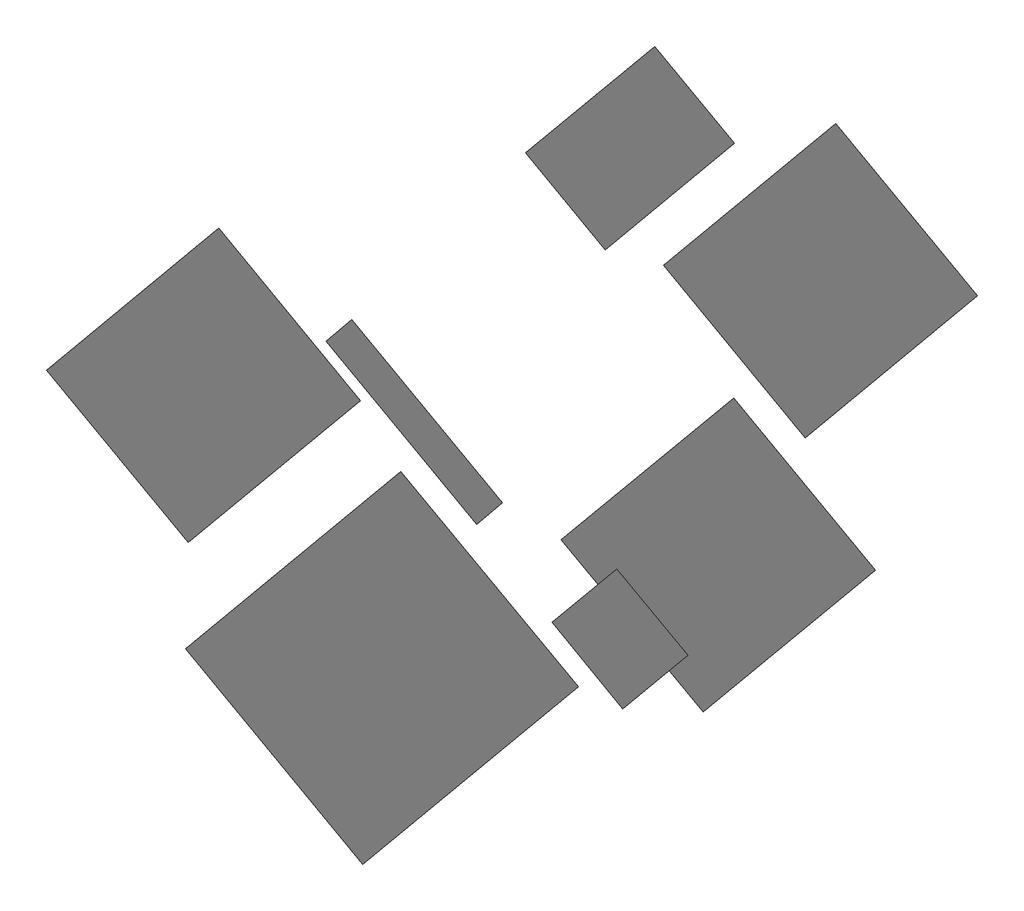
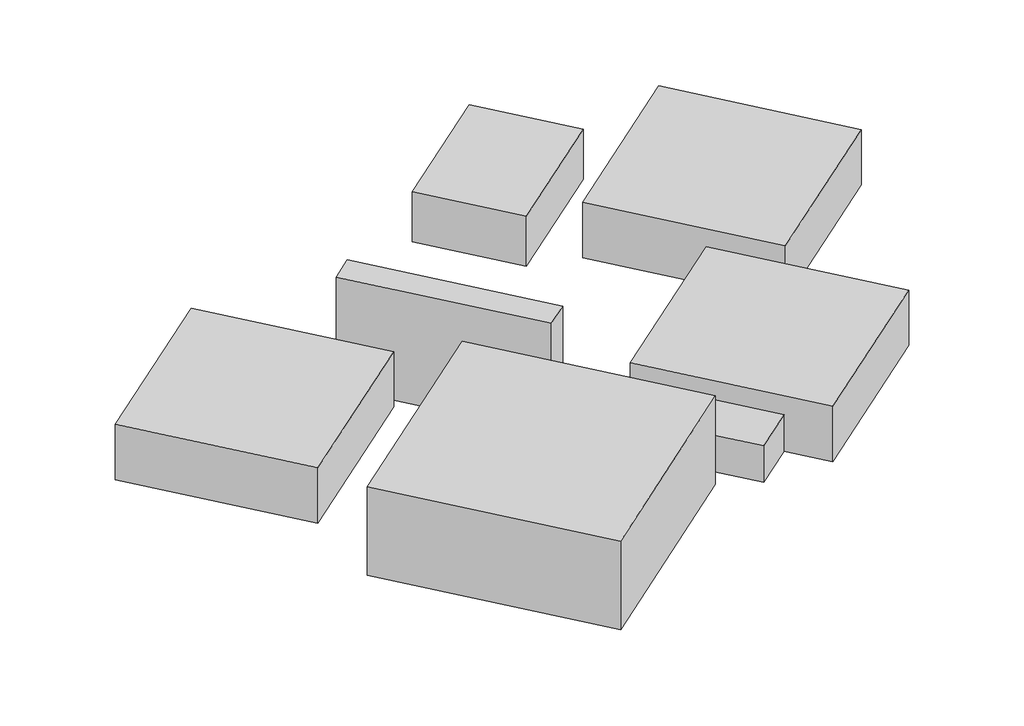
# One storey: 7 proxies.
"""IFC4 building model written with IfcOpenShell, lengths in millimetres."""

from ifc_helpers import new_model, si_unit, frame, origin, place, context, project, spatial, polyline, outline, extrude, element, save

model = new_model("IFC4")

# Units and contexts
model_context = context("Model", 3, world=origin())
ifc_project = project(units=[si_unit("LENGTHUNIT", "METRE", prefix="MILLI")], contexts=[model_context])

# Site, building, storey
site = spatial("IfcSite", under=ifc_project)
building = spatial("IfcBuilding", under=site)
storey = spatial("IfcBuildingStorey", under=building, Name="f2-展厅", Elevation=10300.0)

# Proxies
placement = place(None, origin())
element("IfcBuildingElementProxy", 1, Name="走廊 : 走廊_17米", ObjectType="走廊 : 走廊_17米", at=placement, inside=storey, context=model_context, shape_type="SweptSolid", body=[
    extrude(outline(polyline([(-32285.2445231, 12352.2279231), (-30432.0706072, 13877.2677381), (-19629.7052504, 750.6191675), (-21482.8791663, -774.4206476), (-32285.2445231, 12352.2279231)])), frame((0.0, 0.0, 10300.0), z_axis=(0.0, 0.0, 1.0), x_axis=(1.0, 0.0, 0.0)), (0.0, 0.0, 1.0), 10000.0),
])
element("IfcBuildingElementProxy", 2, Name="公共-封闭 : Gallery-Big", ObjectType="公共-封闭 : Gallery-Big", at=placement, inside=storey, context=model_context, shape_type="SweptSolid", body=[
    extrude(outline(polyline([(-42360.2281464, -9723.9608398), (-26917.1121809, 2984.7042859), (-14208.4470552, -12458.4116796), (-29651.5630207, -25167.0768053), (-42360.2281464, -9723.9608398)])), frame((0.0, 0.0, 10300.0), z_axis=(0.0, 0.0, 1.0), x_axis=(1.0, 0.0, 0.0)), (0.0, 0.0, 1.0), 8000.0),
])
element("IfcBuildingElementProxy", 3, Name="公共-封闭 : Gallery-Middle", ObjectType="公共-封闭 : Gallery-Middle", at=placement, inside=storey, context=model_context, shape_type="SweptSolid", body=[
    extrude(outline(polyline([(2090.836591, 5429.9489753), (-8076.0955096, 17784.4417477), (4278.3972628, 27951.3738482), (14445.3293634, 15596.8810759), (2090.836591, 5429.9489753)])), frame((0.0, 0.0, 10300.0), z_axis=(0.0, 0.0, 1.0), x_axis=(1.0, 0.0, 0.0)), (0.0, 0.0, 1.0), 5000.0),
])
element("IfcBuildingElementProxy", 4, Name="公共-封闭 : Gallery-Middle", ObjectType="公共-封闭 : Gallery-Middle", at=placement, inside=storey, context=model_context, shape_type="SweptSolid", body=[
    extrude(outline(polyline([(-42168.9762252, -2078.413244), (-52335.9083258, 10276.0795284), (-39981.4155534, 20443.0116289), (-29814.4834528, 8088.5188565), (-42168.9762252, -2078.413244)])), frame((0.0, 0.0, 10300.0), z_axis=(0.0, 0.0, 1.0), x_axis=(1.0, 0.0, 0.0)), (0.0, 0.0, 1.0), 5000.0),
])
element("IfcBuildingElementProxy", 5, Name="公共-封闭 : Gallery-Middle", ObjectType="公共-封闭 : Gallery-Middle", at=placement, inside=storey, context=model_context, shape_type="SweptSolid", body=[
    extrude(outline(polyline([(-5228.4607435, -14250.3737471), (-15395.392844, -1895.8809747), (-3040.9000717, 8271.0511259), (7126.0320289, -4083.4416465), (-5228.4607435, -14250.3737471)])), frame((0.0, 0.0, 10300.0), z_axis=(0.0, 0.0, 1.0), x_axis=(1.0, 0.0, 0.0)), (0.0, 0.0, 1.0), 5000.0),
])
element("IfcBuildingElementProxy", 6, Name="公共-封闭 : Gallery-Small", ObjectType="公共-封闭 : Gallery-Small", at=placement, inside=storey, context=model_context, shape_type="SweptSolid", body=[
    extrude(outline(polyline([(-12256.9381005, 18909.0766924), (-17975.8374071, 25858.4788769), (-8709.9678278, 33483.6779523), (-2991.0685212, 26534.2757679), (-12256.9381005, 18909.0766924)])), frame((0.0, 0.0, 10300.0), z_axis=(0.0, 0.0, 1.0), x_axis=(1.0, 0.0, 0.0)), (0.0, 0.0, 1.0), 4500.0),
])
element("IfcBuildingElementProxy", 7, Name="临时私有-封闭 : Restrooms-Gallery-2f", ObjectType="临时私有-封闭 : Restrooms-Gallery-2f", at=placement, inside=storey, context=model_context, shape_type="SweptSolid", body=[
    extrude(outline(polyline([(-6352.7890456, -10193.6386218), (-10985.7238352, -14006.2381595), (-16069.1898855, -7828.9917733), (-11436.2550959, -4016.3922356), (-6352.7890456, -10193.6386218)])), frame((0.0, 0.0, 10300.0), z_axis=(0.0, 0.0, 1.0), x_axis=(1.0, 0.0, 0.0)), (0.0, 0.0, 1.0), 3300.0),
])

save(model, "model.ifc")

# Revit data of these elements
# Type "走廊 : 走廊_17米"
#   Default Elevation = 1219.2 mm
#   公共_流动_空间_进深 [instance default] = 2400 mm
#   公共_流动_空间_开间 [instance default] = 17000 mm
#   公共_流动_空间_层高 [instance default] = 10000 mm
# Type "公共-封闭 : Gallery-Big"
#   Default Elevation = 1219.2 mm
#   公共_封闭_房间_面积 = 400.00 m²
#   公共_封闭_房间_进深 = 20000 mm
#   公共_封闭_房间_开间 = 20000 mm
#   公共_封闭_房间_层高 = 8000 mm
# Type "公共-封闭 : Gallery-Middle"
#   Default Elevation = 1219.2 mm
#   公共_封闭_房间_面积 = 256.00 m²
#   公共_封闭_房间_进深 = 16000 mm
#   公共_封闭_房间_开间 = 16000 mm
#   公共_封闭_房间_层高 = 5000 mm
# Type "公共-封闭 : Gallery-Small"
#   Default Elevation = 1219.2 mm
#   公共_封闭_房间_面积 = 108.00 m²
#   公共_封闭_房间_进深 = 9000 mm
#   公共_封闭_房间_开间 = 12000 mm
#   公共_封闭_房间_层高 = 4500 mm
# Type "临时私有-封闭 : Restrooms-Gallery-2f"
#   Default Elevation = 1219.2 mm
#   临时私有_封闭_房间_面积 = 48.00 m²
#   临时私有_封闭_房间_进深 = 6000 mm
#   临时私有_封闭_房间_开间 = 8000 mm
#   临时私有_封闭_房间_层高 = 3300 mm
# Element 1 (IfcBuildingElementProxy, "走廊 : 走廊_17米")
#   Phase Created = 新构造
#   Materials on its faces: "公共_流动_空间"
# Element 2 (IfcBuildingElementProxy, "公共-封闭 : Gallery-Big")
#   Phase Created = 新构造
#   Materials on its faces: "公共_封闭_房间"
# Elements 3, 4, 5 (IfcBuildingElementProxy, "公共-封闭 : Gallery-Middle")
#   Phase Created = 新构造
#   Materials on its faces: "公共_封闭_房间"
# Element 6 (IfcBuildingElementProxy, "公共-封闭 : Gallery-Small")
#   Phase Created = 新构造
#   Materials on its faces: "公共_封闭_房间"
# Element 7 (IfcBuildingElementProxy, "临时私有-封闭 : Restrooms-Gallery-2f")
#   Phase Created = 新构造
#   Materials on its faces: "临时私有_封闭_房间"
# Materials
#   "公共_流动_空间": class "玻璃", colour RGB 0 0 128, transparency 0.5
#   "公共_封闭_房间": class "其他", colour RGB 135 60 10, transparency 0
#   "临时私有_封闭_房间": class "其他", colour RGB 77 38 0, transparency 0
